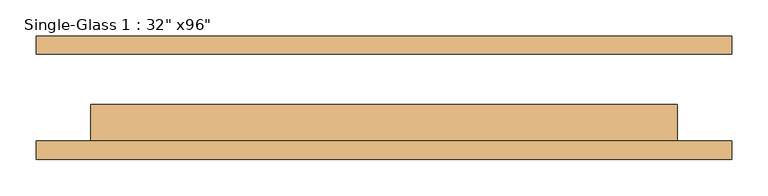
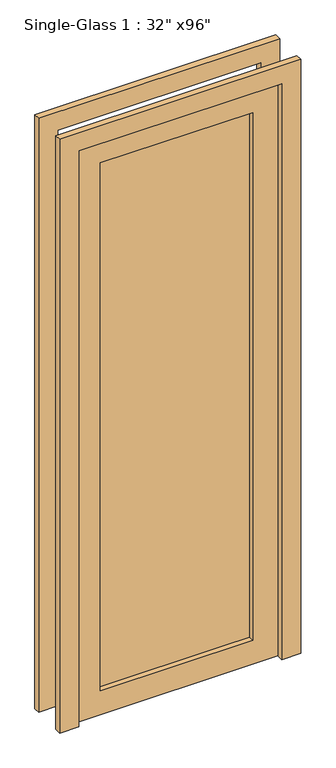
"""IFC4 building model written with IfcOpenShell, lengths in millimetres: door geometry."""

import ifcopenshell
import ifcopenshell.guid

model = None  # the IFC model being written
_history = None  # IfcOwnerHistory: only IFC2X3 demands one
_inside = {}  # id of a spatial element -> (the spatial element, [elements in it])
_under = {}  # id of a project, library or spatial element -> (it, [spatial elements below it])
_declared = {}  # id of a project -> (the project, [libraries it declares])
_typed = {}  # id of a type object -> (the type object, [elements of that type])
_made_of = {}  # id of a material, layer set ... -> (it, [elements and type objects made of it])


def new_model(schema):
    """Start an empty IFC model of exactly this schema.

    Asked for "IFC4X3", IfcOpenShell would pick the latest addendum, in which some entities
    have other attributes; the version numbers below select the first issue.
    IFC2X3 requires an IfcOwnerHistory on every rooted entity: one is made here for all.
    """
    global model, _history
    if schema == "IFC4X3":
        model = ifcopenshell.file(schema_version=(4, 3, 0, 0))
    else:
        model = ifcopenshell.file(schema=schema)
    _inside.clear()
    _under.clear()
    _declared.clear()
    _typed.clear()
    _made_of.clear()
    _history = None
    if model.schema == "IFC2X3":
        org = make("IfcOrganization", Name="unknown")
        user = make(
            "IfcPersonAndOrganization",
            ThePerson=make("IfcPerson", FamilyName="unknown"),
            TheOrganization=org,
        )
        app = make(
            "IfcApplication",
            ApplicationDeveloper=org,
            Version="unknown",
            ApplicationFullName="unknown",
            ApplicationIdentifier="unknown",
        )
        _history = make(
            "IfcOwnerHistory",
            OwningUser=user,
            OwningApplication=app,
            ChangeAction="ADDED",
            CreationDate=0,
        )
    return model


def make(cls, **values):
    """One entity of the class cls with the attributes given. An attribute that is None is left unset."""
    return model.create_entity(
        cls, **{name: value for name, value in values.items() if value is not None}
    )


def rooted(cls, **values):
    """An entity with a GlobalId (a new one), such as an element, a storey or a relation."""
    return make(cls, GlobalId=ifcopenshell.guid.new(), OwnerHistory=_history, **values)


def si_unit(unit_type, name, prefix=None):
    """IfcSIUnit, for example si_unit("LENGTHUNIT", "METRE", prefix="MILLI")."""
    return make("IfcSIUnit", UnitType=unit_type, Prefix=prefix, Name=name)


def assignment(units):
    """IfcUnitAssignment: the units of a project."""
    return None if units is None else make("IfcUnitAssignment", Units=units)


def point(xyz):
    """IfcCartesianPoint."""
    return None if xyz is None else make("IfcCartesianPoint", Coordinates=xyz)


def direction(xyz):
    """IfcDirection."""
    return None if xyz is None else make("IfcDirection", DirectionRatios=xyz)


def frame(location, z_axis=None, x_axis=None):
    """IfcAxis2Placement3D, a coordinate frame: its origin and axes. An axis left out is left unset."""
    return make(
        "IfcAxis2Placement3D",
        Location=point(location),
        Axis=direction(z_axis),
        RefDirection=direction(x_axis),
    )


def origin():
    """The frame at (0, 0, 0) with its axes left unset."""
    return frame((0.0, 0.0, 0.0))


def place(relative_to, where):
    """IfcLocalPlacement: puts the frame where relative to a parent placement (None: the world)."""
    return make(
        "IfcLocalPlacement", PlacementRelTo=relative_to, RelativePlacement=where
    )


def context(
    kind, dimensions, precision=None, world=None, true_north=None, identifier=None
):
    """IfcGeometricRepresentationContext, for example the 3D "Model" context."""
    return make(
        "IfcGeometricRepresentationContext",
        ContextIdentifier=identifier,
        ContextType=kind,
        CoordinateSpaceDimension=dimensions,
        Precision=precision,
        WorldCoordinateSystem=world,
        TrueNorth=true_north,
    )


def project(units=None, contexts=None):
    """IfcProject with its units and contexts."""
    return rooted(
        "IfcProject",
        Name="project",
        RepresentationContexts=contexts,
        UnitsInContext=assignment(units),
    )


def spatial(cls, under=None, at=None, **own):
    """A site, building, storey or space (cls), placed at a placement, below another one or the project."""
    s = rooted(cls, ObjectPlacement=at, **own)
    if under is not None:
        _under.setdefault(under.id(), (under, []))[1].append(s)
    return s


def polyline(points):
    """IfcPolyline through the points."""
    return make("IfcPolyline", Points=[point(p) for p in points])


def outline(outer, holes=None, kind="AREA"):
    """IfcArbitraryClosedProfileDef: a profile drawn as a closed curve; with holes, ...WithVoids."""
    if holes is None:
        return make("IfcArbitraryClosedProfileDef", ProfileType=kind, OuterCurve=outer)
    return make(
        "IfcArbitraryProfileDefWithVoids",
        ProfileType=kind,
        OuterCurve=outer,
        InnerCurves=holes,
    )


def extrude(swept, where, along, depth):
    """IfcExtrudedAreaSolid: the profile swept, set in the frame where, extruded along a direction by depth."""
    return make(
        "IfcExtrudedAreaSolid",
        SweptArea=swept,
        Position=where,
        ExtrudedDirection=direction(along),
        Depth=depth,
    )


def shape(context_of_items, identifier, shape_type, items):
    """IfcShapeRepresentation: the items that make up one representation, for example the "Body"."""
    return make(
        "IfcShapeRepresentation",
        ContextOfItems=context_of_items,
        RepresentationIdentifier=identifier,
        RepresentationType=shape_type,
        Items=items,
    )


def source(mapping_origin, context_of_items, identifier, shape_type, items):
    """IfcRepresentationMap: a shape defined once, which mapped items show again and again."""
    return make(
        "IfcRepresentationMap",
        MappingOrigin=mapping_origin,
        MappedRepresentation=shape(context_of_items, identifier, shape_type, items),
    )


def transform(
    local_origin,
    x_axis=None,
    y_axis=None,
    z_axis=None,
    scale=None,
    scale2=None,
    scale3=None,
    uniform=True,
):
    """IfcCartesianTransformationOperator3D, or its non-uniform kind. x_axis, y_axis, z_axis: its Axis1, 2, 3."""
    if uniform:
        return make(
            "IfcCartesianTransformationOperator3D",
            Axis1=direction(x_axis),
            Axis2=direction(y_axis),
            LocalOrigin=point(local_origin),
            Scale=scale,
            Axis3=direction(z_axis),
        )
    return make(
        "IfcCartesianTransformationOperator3DnonUniform",
        Axis1=direction(x_axis),
        Axis2=direction(y_axis),
        LocalOrigin=point(local_origin),
        Scale=scale,
        Axis3=direction(z_axis),
        Scale2=scale2,
        Scale3=scale3,
    )


def mapped(mapping_source, mapping_target):
    """IfcMappedItem: shows the shape of a source again, moved by a transform."""
    return make(
        "IfcMappedItem", MappingSource=mapping_source, MappingTarget=mapping_target
    )


def made_of(thing, what):
    """Note that an element or type object is made of a material, layer set ...; save() writes the relation."""
    if what is not None:
        _made_of.setdefault(what.id(), (what, []))[1].append(thing)
    return thing


def element(
    cls,
    number,
    at=None,
    inside=None,
    cuts=None,
    type_object=None,
    material=None,
    context=None,
    identifier="Body",
    shape_type=None,
    held_by="IfcProductDefinitionShape",
    body=None,
    shapes=None,
    **own,
):
    """One element of the class cls, such as IfcWall. Its Tag is "e" and its number.

    at: its placement. inside: the storey or other place that contains it. cuts: it is an
    opening in that element (IfcRelVoidsElement). A single representation is given by context,
    identifier, shape_type and body (its items); several are given by shapes. held_by: the class
    of the entity that holds the representations. save() writes the other relations.
    """
    e = rooted(cls, Tag="e%d" % number, ObjectPlacement=at, **own)
    if body is not None:
        shapes = [shape(context, identifier, shape_type, body)]
    if shapes is not None:
        e.Representation = make(held_by, Representations=shapes)
    if inside is not None:
        _inside.setdefault(inside.id(), (inside, []))[1].append(e)
    if cuts is not None:
        rooted(
            "IfcRelVoidsElement", RelatingBuildingElement=cuts, RelatedOpeningElement=e
        )
    if type_object is not None:
        _typed.setdefault(type_object.id(), (type_object, []))[1].append(e)
    return made_of(e, material)


def aggregate(whole, parts):
    """IfcRelAggregates: a whole, such as a stair, and the parts it consists of."""
    return rooted("IfcRelAggregates", RelatingObject=whole, RelatedObjects=parts)


def save(model, path):
    """Write the relations noted so far, then the file.

    IfcRelAggregates (storeys below a building ...), IfcRelContainedInSpatialStructure (elements
    in a storey), IfcRelDefinesByType, IfcRelAssociatesMaterial and IfcRelDeclares: one each for
    every whole, place, type object, material and project.
    """
    for whole, parts in _under.values():
        aggregate(whole, parts)
    for where, things in _inside.values():
        rooted(
            "IfcRelContainedInSpatialStructure",
            RelatedElements=things,
            RelatingStructure=where,
        )
    for kind, things in _typed.values():
        rooted("IfcRelDefinesByType", RelatedObjects=things, RelatingType=kind)
    for what, things in _made_of.values():
        rooted("IfcRelAssociatesMaterial", RelatedObjects=things, RelatingMaterial=what)
    for by, libraries in _declared.values():
        rooted("IfcRelDeclares", RelatingContext=by, RelatedDefinitions=libraries)
    model.write(path)


def door_4b229a85(model_context):
    return source(origin(), model_context, "Body", "SweptSolid", [
        extrude(outline(polyline([(2438.4, 406.4), (0.0, 406.4), (0.0, 482.6), (2514.6, 482.6), (2514.6, -482.6), (0.0, -482.6), (0.0, -406.4), (2438.4, -406.4), (2438.4, 406.4)])), frame((0.0, 60.325, 0.0), z_axis=(0.0, 1.0, 0.0), x_axis=(0.0, 0.0, 1.0)), (0.0, 0.0, 1.0), 25.4),
        extrude(outline(polyline([(2438.4, 406.4), (0.0, 406.4), (0.0, 482.6), (2514.6, 482.6), (2514.6, -482.6), (0.0, -482.6), (0.0, -406.4), (2438.4, -406.4), (2438.4, 406.4)])), frame((0.0, -85.725, 0.0), z_axis=(0.0, 1.0, 0.0), x_axis=(0.0, 0.0, 1.0)), (0.0, 0.0, 1.0), 25.4),
        extrude(outline(polyline([(304.8, -31.75), (304.8, -38.1), (-304.8, -38.1), (-304.8, -31.75), (304.8, -31.75)])), frame((0.0, 0.0, 101.6), z_axis=(0.0, 0.0, 1.0), x_axis=(1.0, 0.0, 0.0)), (0.0, 0.0, 1.0), 2235.2),
        extrude(outline(polyline([(2438.4, 406.4), (2438.4, -406.4), (0.0, -406.4), (0.0, 406.4), (2438.4, 406.4)]), holes=[polyline([(2336.8, -304.8), (2336.8, 304.8), (101.6, 304.8), (101.6, -304.8), (2336.8, -304.8)])]), frame((0.0, -60.325, 0.0), z_axis=(0.0, 1.0, 0.0), x_axis=(0.0, 0.0, 1.0)), (0.0, 0.0, 1.0), 50.8),
    ])


if __name__ == "__main__":
    model = new_model("IFC4")
    model_context = context("Model", 3, world=origin())
    ifc_project = project(units=[si_unit("LENGTHUNIT", "METRE", prefix="MILLI")], contexts=[model_context])
    site = spatial("IfcSite", under=ifc_project)
    building = spatial("IfcBuilding", under=site)
    placement = place(None, origin())
    door_shape = door_4b229a85(model_context)
    element("IfcDoor", 1, ObjectType="Single-Glass 1 : 32\" x96\"", at=placement, inside=building, context=model_context, shape_type="MappedRepresentation", body=[
        mapped(door_shape, transform((0.0, 0.0, 0.0), x_axis=(1.0, 0.0, 0.0), y_axis=(0.0, 1.0, 0.0), z_axis=(0.0, 0.0, 1.0))),
    ])
    save(model, "model.ifc")

# Revit data of these elements
# Type "Single-Glass 1 : 32\" x96\""
#   Type Mark = "31"
#   Construction Type Id = "MDOOR"
#   Assembly Code = "C1020"
#   Analytic Construction = "Metal"
#   Thickness = 0' - 2"
#   Heat Transfer Coefficient (U) = 3.7021 W/(m²·K)
#   Height = 8' - 0"
#   Rail Width - Base = 0' - 4"
#   Rail Width - Top = 0' - 4"
#   Stile Width - Hinge = 0' - 4"
#   Stile Width - Latch = 0' - 4"
#   Trim Projection Ext = 0' - 1"
#   Trim Projection Int = 0' - 1"
#   Trim Width = 0' - 3"
#   Width = 2' - 8"
#   Door Material = Aluminum
#   Frame Material = Aluminum
#   Visual Light Transmittance = 0
#   Solar Heat Gain Coefficient = 0
#   Function = (empty or 0)
#   Wall Closure = (empty or 0)
# Element 1 (IfcDoor, "Single-Glass 1 : 32\" x96\"")
#   Materials on its faces: "Aluminum", "Glass"
# Materials
#   "Aluminum": class "Metal", colour RGB 226 226 226, transparency 0, Description = "Aluminum 6061", Cost = 0
#   "Glass": class "Glass", colour RGB 142 168 196, transparency 0.75, Description = "Soda Lime Glass", Cost = 0
